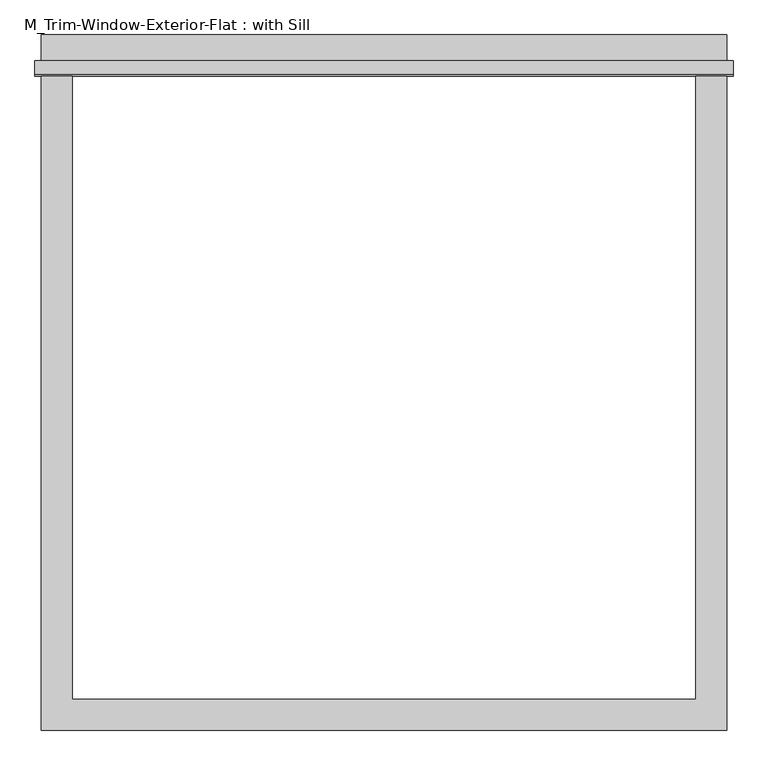
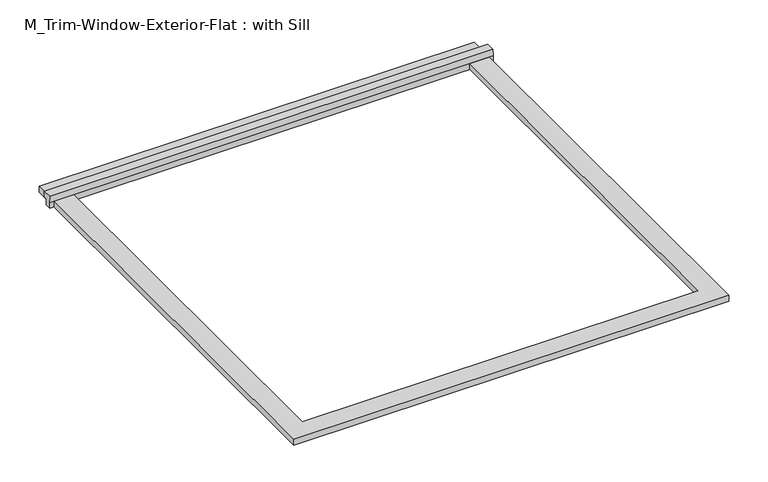
"""IFC4 building model written with IfcOpenShell, lengths in millimetres: proxy geometry, M_Trim-Window-Exterior-Flat : with Sill."""

from ifc_helpers import new_model, si_unit, frame, origin, origin_with_axes, place, context, project, spatial, polyline, outline, extrude, source, transform, mapped, element, save


def m_trim_window_exterior_flat_with_sill_8c23e1cb(model_context):
    return source(origin(), model_context, "Body", "SweptSolid", [
        extrude(outline(polyline([(669.6, 1239.6323709), (-669.6, 1239.6323709), (-669.6, 1299.6323709), (669.6, 1299.6323709), (669.6, 1239.6323709)])), origin_with_axes(), (0.0, 0.0, 1.0), 19.05),
        extrude(outline(polyline([(1249.2, 38.1), (1249.2, 19.05), (1239.6323709, 19.05), (1239.6323709, 0.0), (1219.2, 0.0), (1219.2, 19.05), (1221.6580645, 38.1), (1249.2, 38.1)])), frame((-682.3, 0.0, 0.0), z_axis=(1.0, 0.0, 0.0), x_axis=(0.0, 1.0, 0.0)), (0.0, 0.0, 1.0), 1364.6),
        extrude(outline(polyline([(-669.6, -60.0), (-669.6, 1219.2), (-609.6, 1219.2), (-609.6, 0.0), (609.6, 0.0), (609.6, 1219.2), (669.6, 1219.2), (669.6, -60.0), (-669.6, -60.0)])), origin_with_axes(), (0.0, 0.0, 1.0), 19.05),
    ])


if __name__ == "__main__":
    model = new_model("IFC4")
    model_context = context("Model", 3, world=origin())
    ifc_project = project(units=[si_unit("LENGTHUNIT", "METRE", prefix="MILLI")], contexts=[model_context])
    site = spatial("IfcSite", under=ifc_project)
    building = spatial("IfcBuilding", under=site)
    placement = place(None, origin())
    m_trim_window_exterior_flat_with_sill_shape = m_trim_window_exterior_flat_with_sill_8c23e1cb(model_context)
    element("IfcBuildingElementProxy", 1, Name="M_Trim-Window-Exterior-Flat : with Sill", ObjectType="M_Trim-Window-Exterior-Flat : with Sill", at=placement, inside=building, context=model_context, shape_type="MappedRepresentation", body=[
        mapped(m_trim_window_exterior_flat_with_sill_shape, transform((0.0, 0.0, 0.0), x_axis=(1.0, 0.0, 0.0), y_axis=(0.0, 1.0, 0.0), z_axis=(0.0, 0.0, 1.0))),
    ])
    save(model, "model.ifc")

# Revit data of these elements
# Type "M_Trim-Window-Exterior-Flat : with Sill"
#   Trim Width = 0' - 2.3622"
#   Trim Thickness_Picture Frame = 0' - 1.1811"
#   Trim Thickness_with Sill = 0' - 0 3/4"
#   Sill Thickness = 0' - 1.1811"
#   Opening Width [instance default] = 1' - 11.62205"
#   Opening Height [instance default] = 2' - 11.43307"
#   Default Elevation = 3' - 11.24409"
#   Sill = yes
#   Picture Frame = no
#   Trim Material [instance default] = none
# Element 1 (IfcBuildingElementProxy, "M_Trim-Window-Exterior-Flat : with Sill")
#   Opening Width = 4' - 0"
#   Opening Height = 4' - 0"
#   Trim Material = Clad - White
#   Materials on its faces: "Clad - White"
# Materials
#   "Clad - White": class "Wood", colour RGB 242 242 238, transparency 0, Cost = 0
